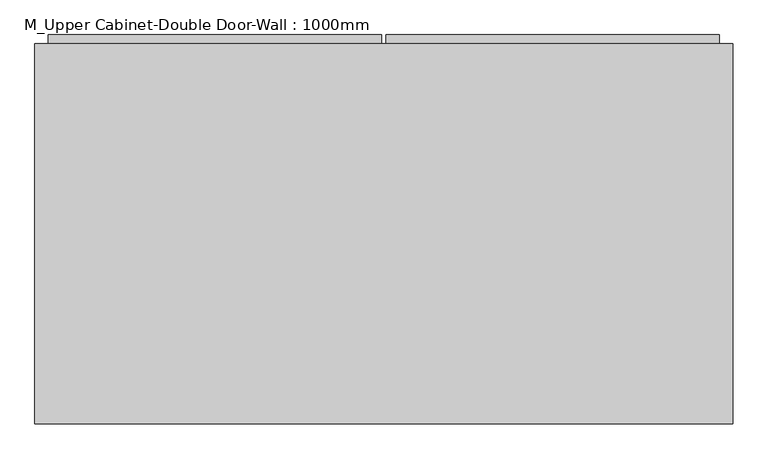
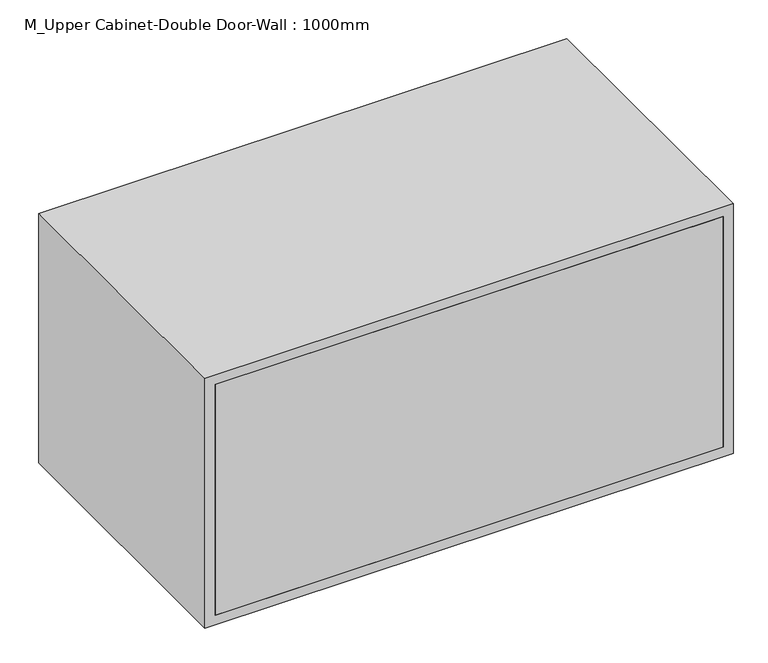
"""IFC4 building model written with IfcOpenShell, lengths in millimetres: furniture geometry, M_Upper Cabinet-Double Door-Wall : 1000mm."""

from ifc_helpers import new_model, si_unit, frame, origin, place, context, project, spatial, polyline, outline, extrude, source, transform, mapped, element, save


def m_upper_cabinet_double_door_wall_1000mm_1530bdee(model_context):
    return source(origin(), model_context, "Body", "SweptSolid", [
        extrude(outline(polyline([(32.9461628, 645.2), (510.7211628, 645.2), (510.7211628, 613.45), (32.9461628, 613.45), (32.9461628, 645.2)])), frame((0.0, 0.0, 119.05), z_axis=(0.0, 0.0, 1.0), x_axis=(1.0, 0.0, 0.0)), (0.0, 0.0, 1.0), 461.9),
        extrude(outline(polyline([(-451.1788372, 645.2), (26.5961628, 645.2), (26.5961628, 613.45), (-451.1788372, 613.45), (-451.1788372, 645.2)])), frame((0.0, 0.0, 119.05), z_axis=(0.0, 0.0, 1.0), x_axis=(1.0, 0.0, 0.0)), (0.0, 0.0, 1.0), 461.9),
        extrude(outline(polyline([(510.7211628, 87.5), (-451.1788372, 87.5), (-451.1788372, 106.55), (510.7211628, 106.55), (510.7211628, 87.5)])), frame((0.0, 0.0, 119.05), z_axis=(0.0, 0.0, 1.0), x_axis=(1.0, 0.0, 0.0)), (0.0, 0.0, 1.0), 461.9),
        extrude(outline(polyline([(600.0, -470.2288372), (100.0, -470.2288372), (100.0, 529.7711628), (600.0, 529.7711628), (600.0, -470.2288372)]), holes=[polyline([(580.95, -451.1788372), (580.95, 510.7211628), (119.05, 510.7211628), (119.05, -451.1788372), (580.95, -451.1788372)])]), frame((0.0, 87.5, 0.0), z_axis=(0.0, 1.0, 0.0), x_axis=(0.0, 0.0, 1.0)), (0.0, 0.0, 1.0), 545.0),
    ])


if __name__ == "__main__":
    model = new_model("IFC4")
    model_context = context("Model", 3, world=origin())
    ifc_project = project(units=[si_unit("LENGTHUNIT", "METRE", prefix="MILLI")], contexts=[model_context])
    site = spatial("IfcSite", under=ifc_project)
    building = spatial("IfcBuilding", under=site)
    placement = place(None, origin())
    m_upper_cabinet_double_door_wall_1000mm_shape = m_upper_cabinet_double_door_wall_1000mm_1530bdee(model_context)
    element("IfcFurniture", 1, ObjectType="M_Upper Cabinet-Double Door-Wall : 1000mm", at=placement, inside=building, context=model_context, shape_type="MappedRepresentation", body=[
        mapped(m_upper_cabinet_double_door_wall_1000mm_shape, transform((0.0, 0.0, 0.0), x_axis=(1.0, 0.0, 0.0), y_axis=(0.0, 1.0, 0.0), z_axis=(0.0, 0.0, 1.0))),
    ])
    save(model, "model.ifc")

# Revit data of these elements
# Type "M_Upper Cabinet-Double Door-Wall : 1000mm"
#   COBie.Type.CreatedBy = "design@eagle.com"
#   COBie.Type.CreatedOn = "2016-09-01T06:50:21"
#   COBie.Type.Name = "Casework_M_Upper Cabinet-Double Door-Wall_1000mm"
#   COBie.Type.Category = "23-40 35 17 47 11 : Kitchen Casework"
#   COBie.Type.Description = ""
#   COBie.Type.Manufacturer = ""
#   COBie.Type.ModelNumber = ""
#   COBie.Type.ReplacementCost = 0
#   Depth = 545 mm
#   Height = 500 mm
#   Top Of Cabinet = 600 mm
#   Width = 1000 mm
#   COBie.Type = no
#   Cabinet Material = Door - Panel
#   Door/Drawer Material = Door - Panel
#   Handle Material = Cabinets - Handles
# Element 1 (IfcFurniture, "M_Upper Cabinet-Double Door-Wall : 1000mm")
#   Materials on its faces: "Door - Panel"
# Materials
#   "Door - Panel": class "Wood", colour RGB 210 159 95, transparency 0
#   "Cabinets - Handles": class "Metal", colour RGB 57 57 57, transparency 0
